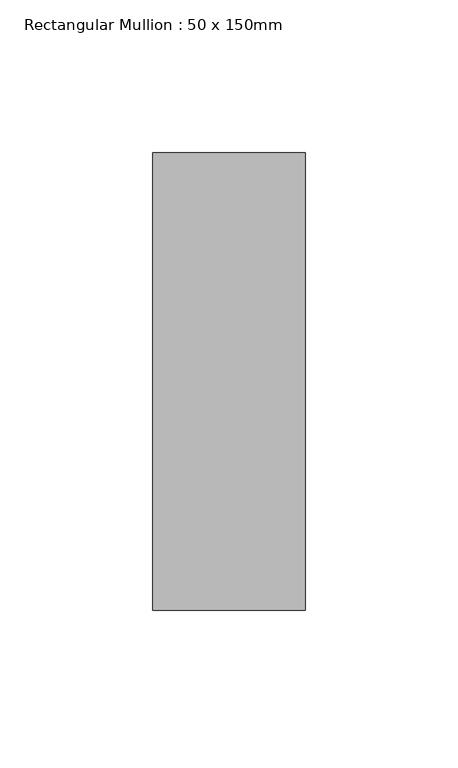
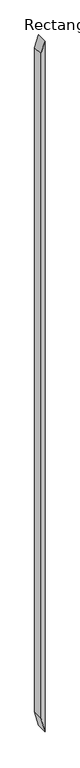
"""IFC4 building model written with IfcOpenShell, lengths in millimetres: member geometry, Rectangular Mullion : 50 x 150mm."""

from ifc_helpers import new_model, si_unit, frame, origin, place, context, project, spatial, polyline, outline, extrude, source, transform, mapped, element, save


def rectangular_mullion_50_x_150mm_375b3459(model_context):
    return source(origin(), model_context, "Body", "SweptSolid", [
        extrude(outline(polyline([(0.0, 0.0), (-161.7316361, -50.0), (-9569.8514431, -50.0), (-9783.1614006, 0.0), (0.0, 0.0)])), frame((0.0, -75.0, 0.0), z_axis=(0.0, 1.0, 0.0), x_axis=(0.0, 0.0, 1.0)), (0.0, 0.0, 1.0), 150.0),
    ])


if __name__ == "__main__":
    model = new_model("IFC4")
    model_context = context("Model", 3, world=origin())
    ifc_project = project(units=[si_unit("LENGTHUNIT", "METRE", prefix="MILLI")], contexts=[model_context])
    site = spatial("IfcSite", under=ifc_project)
    building = spatial("IfcBuilding", under=site)
    placement = place(None, origin())
    rectangular_mullion_50_x_150mm_shape = rectangular_mullion_50_x_150mm_375b3459(model_context)
    element("IfcMember", 1, ObjectType="Rectangular Mullion : 50 x 150mm", at=placement, inside=building, context=model_context, shape_type="MappedRepresentation", body=[
        mapped(rectangular_mullion_50_x_150mm_shape, transform((0.0, 0.0, 0.0), x_axis=(1.0, 0.0, 0.0), y_axis=(0.0, 1.0, 0.0), z_axis=(0.0, 0.0, 1.0))),
    ])
    save(model, "model.ifc")

# Revit data of these elements
# Type "Rectangular Mullion : 50 x 150mm"
#   built-in parameter 1007304 = 0.492126 (stored number, unit not read)
#   built-in parameter 1007301 = 0.082021 (stored number, unit not read)
#   built-in parameter 1007300 = 0.082021 (stored number, unit not read)
# Element 1 (IfcMember, "Rectangular Mullion : 50 x 150mm")
#   Materials on its faces: "Metal - Aluminium"
# Materials
#   "Metal - Aluminium": class "Metal", colour RGB 247 247 247, transparency 0
